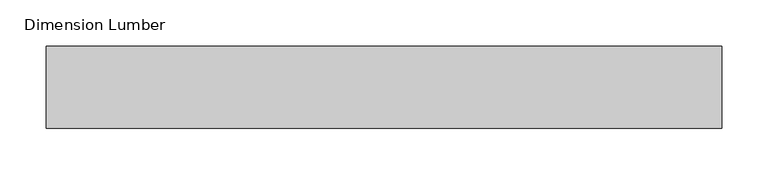
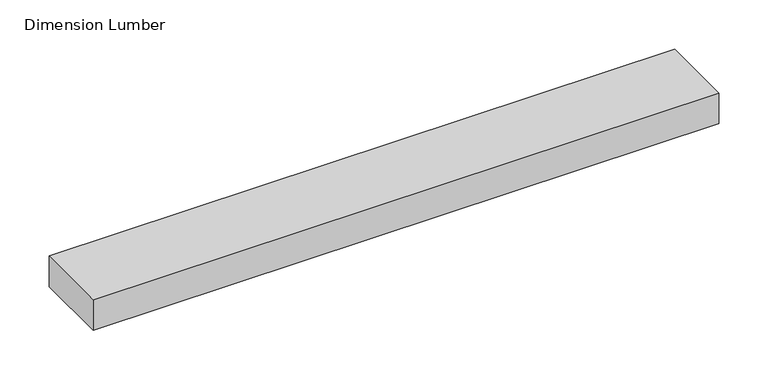
"""IFC4 building model written with IfcOpenShell, lengths in millimetres: beam geometry, Dimension Lumber : Top Supporting Lumbers."""

from ifc_helpers import new_model, si_unit, frame, origin, place, context, project, spatial, polyline, outline, extrude, source, transform, mapped, element, save


def dimension_lumber_348b767d(model_context):
    return source(origin(), model_context, "Body", "SweptSolid", [
        extrude(outline(polyline([(320.675, 44.45), (320.675, -44.45), (-409.575, -44.45), (-409.575, 44.45), (320.675, 44.45)])), frame((0.0, 0.0, -19.05), z_axis=(0.0, 0.0, 1.0), x_axis=(1.0, 0.0, 0.0)), (0.0, 0.0, 1.0), 38.1),
    ])


if __name__ == "__main__":
    model = new_model("IFC4")
    model_context = context("Model", 3, world=origin())
    ifc_project = project(units=[si_unit("LENGTHUNIT", "METRE", prefix="MILLI")], contexts=[model_context])
    site = spatial("IfcSite", under=ifc_project)
    building = spatial("IfcBuilding", under=site)
    placement = place(None, origin())
    dimension_lumber_shape = dimension_lumber_348b767d(model_context)
    element("IfcBeam", 1, ObjectType="Dimension Lumber : Top Supporting Lumbers", at=placement, inside=building, context=model_context, shape_type="MappedRepresentation", body=[
        mapped(dimension_lumber_shape, transform((0.0, 0.0, 0.0), x_axis=(1.0, 0.0, 0.0), y_axis=(0.0, 1.0, 0.0), z_axis=(0.0, 0.0, 1.0))),
    ])
    save(model, "model.ifc")

# Revit data of these elements
# Type "Dimension Lumber : Top Supporting Lumbers"
#   Assembly Code = "B10"
#   A = 0.0364583 SF
#   Length [instance default] = 5' - 0"
#   b = 0' - 3 1/2"
#   d = 0' - 1 1/2"
#   Structural Material [instance default] = Softwood, Lumber
# Element 1 (IfcBeam, "Dimension Lumber : Top Supporting Lumbers")
#   Structural Material = Douglas Fir #2
#   Materials on its faces: "Douglas Fir #2"
# Materials
#   "Softwood, Lumber": class "Wood", colour RGB 223 192 134, transparency 0, Description = "Pinus Echinata", Cost = 0
#   "Douglas Fir #2": class "Wood", colour RGB 223 192 134, transparency 0, Description = "Pinus Echinata", Cost = 0
